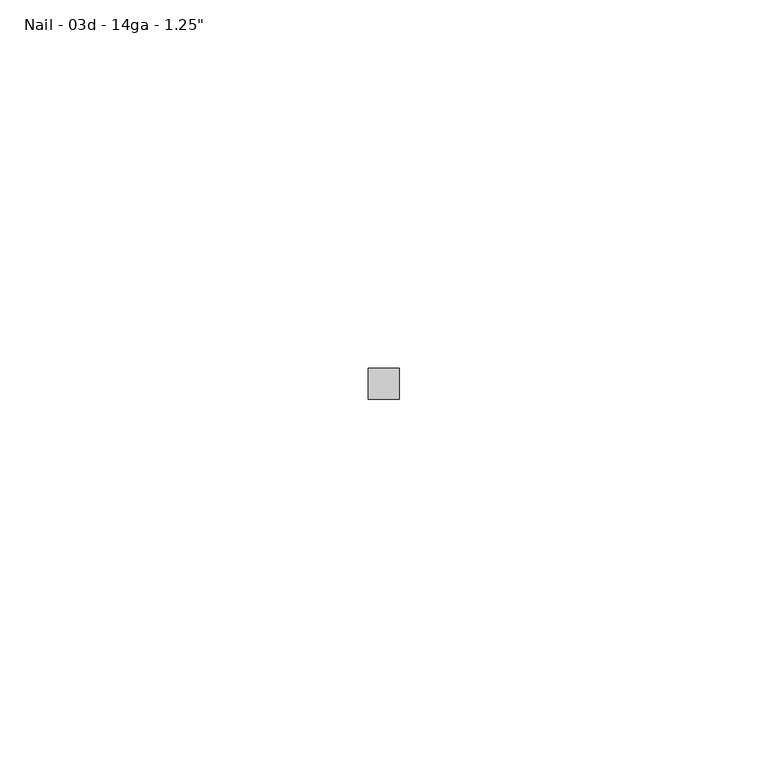
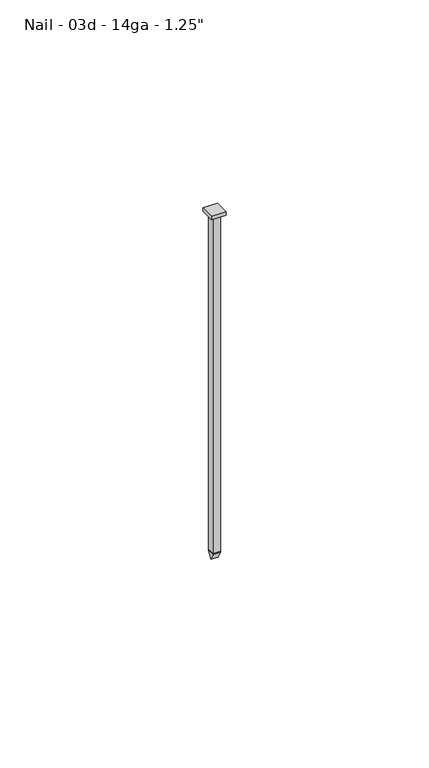
"""IFC4 building model written with IfcOpenShell, lengths in millimetres: fastener geometry."""

import ifcopenshell
import ifcopenshell.guid

model = None  # the IFC model being written
_history = None  # IfcOwnerHistory: only IFC2X3 demands one
_inside = {}  # id of a spatial element -> (the spatial element, [elements in it])
_under = {}  # id of a project, library or spatial element -> (it, [spatial elements below it])
_declared = {}  # id of a project -> (the project, [libraries it declares])
_typed = {}  # id of a type object -> (the type object, [elements of that type])
_made_of = {}  # id of a material, layer set ... -> (it, [elements and type objects made of it])


def new_model(schema):
    """Start an empty IFC model of exactly this schema.

    Asked for "IFC4X3", IfcOpenShell would pick the latest addendum, in which some entities
    have other attributes; the version numbers below select the first issue.
    IFC2X3 requires an IfcOwnerHistory on every rooted entity: one is made here for all.
    """
    global model, _history
    if schema == "IFC4X3":
        model = ifcopenshell.file(schema_version=(4, 3, 0, 0))
    else:
        model = ifcopenshell.file(schema=schema)
    _inside.clear()
    _under.clear()
    _declared.clear()
    _typed.clear()
    _made_of.clear()
    _history = None
    if model.schema == "IFC2X3":
        org = make("IfcOrganization", Name="unknown")
        user = make(
            "IfcPersonAndOrganization",
            ThePerson=make("IfcPerson", FamilyName="unknown"),
            TheOrganization=org,
        )
        app = make(
            "IfcApplication",
            ApplicationDeveloper=org,
            Version="unknown",
            ApplicationFullName="unknown",
            ApplicationIdentifier="unknown",
        )
        _history = make(
            "IfcOwnerHistory",
            OwningUser=user,
            OwningApplication=app,
            ChangeAction="ADDED",
            CreationDate=0,
        )
    return model


def make(cls, **values):
    """One entity of the class cls with the attributes given. An attribute that is None is left unset."""
    return model.create_entity(
        cls, **{name: value for name, value in values.items() if value is not None}
    )


def rooted(cls, **values):
    """An entity with a GlobalId (a new one), such as an element, a storey or a relation."""
    return make(cls, GlobalId=ifcopenshell.guid.new(), OwnerHistory=_history, **values)


def si_unit(unit_type, name, prefix=None):
    """IfcSIUnit, for example si_unit("LENGTHUNIT", "METRE", prefix="MILLI")."""
    return make("IfcSIUnit", UnitType=unit_type, Prefix=prefix, Name=name)


def assignment(units):
    """IfcUnitAssignment: the units of a project."""
    return None if units is None else make("IfcUnitAssignment", Units=units)


def point(xyz):
    """IfcCartesianPoint."""
    return None if xyz is None else make("IfcCartesianPoint", Coordinates=xyz)


def direction(xyz):
    """IfcDirection."""
    return None if xyz is None else make("IfcDirection", DirectionRatios=xyz)


def frame(location, z_axis=None, x_axis=None):
    """IfcAxis2Placement3D, a coordinate frame: its origin and axes. An axis left out is left unset."""
    return make(
        "IfcAxis2Placement3D",
        Location=point(location),
        Axis=direction(z_axis),
        RefDirection=direction(x_axis),
    )


def origin():
    """The frame at (0, 0, 0) with its axes left unset."""
    return frame((0.0, 0.0, 0.0))


def origin_with_axes():
    """The frame at (0, 0, 0) with the z axis (0, 0, 1) and the x axis (1, 0, 0) written out."""
    return frame((0.0, 0.0, 0.0), z_axis=(0.0, 0.0, 1.0), x_axis=(1.0, 0.0, 0.0))


def place(relative_to, where):
    """IfcLocalPlacement: puts the frame where relative to a parent placement (None: the world)."""
    return make(
        "IfcLocalPlacement", PlacementRelTo=relative_to, RelativePlacement=where
    )


def context(
    kind, dimensions, precision=None, world=None, true_north=None, identifier=None
):
    """IfcGeometricRepresentationContext, for example the 3D "Model" context."""
    return make(
        "IfcGeometricRepresentationContext",
        ContextIdentifier=identifier,
        ContextType=kind,
        CoordinateSpaceDimension=dimensions,
        Precision=precision,
        WorldCoordinateSystem=world,
        TrueNorth=true_north,
    )


def project(units=None, contexts=None):
    """IfcProject with its units and contexts."""
    return rooted(
        "IfcProject",
        Name="project",
        RepresentationContexts=contexts,
        UnitsInContext=assignment(units),
    )


def spatial(cls, under=None, at=None, **own):
    """A site, building, storey or space (cls), placed at a placement, below another one or the project."""
    s = rooted(cls, ObjectPlacement=at, **own)
    if under is not None:
        _under.setdefault(under.id(), (under, []))[1].append(s)
    return s


def polyline(points):
    """IfcPolyline through the points."""
    return make("IfcPolyline", Points=[point(p) for p in points])


def outline(outer, holes=None, kind="AREA"):
    """IfcArbitraryClosedProfileDef: a profile drawn as a closed curve; with holes, ...WithVoids."""
    if holes is None:
        return make("IfcArbitraryClosedProfileDef", ProfileType=kind, OuterCurve=outer)
    return make(
        "IfcArbitraryProfileDefWithVoids",
        ProfileType=kind,
        OuterCurve=outer,
        InnerCurves=holes,
    )


def extrude(swept, where, along, depth):
    """IfcExtrudedAreaSolid: the profile swept, set in the frame where, extruded along a direction by depth."""
    return make(
        "IfcExtrudedAreaSolid",
        SweptArea=swept,
        Position=where,
        ExtrudedDirection=direction(along),
        Depth=depth,
    )


def shape(context_of_items, identifier, shape_type, items):
    """IfcShapeRepresentation: the items that make up one representation, for example the "Body"."""
    return make(
        "IfcShapeRepresentation",
        ContextOfItems=context_of_items,
        RepresentationIdentifier=identifier,
        RepresentationType=shape_type,
        Items=items,
    )


def source(mapping_origin, context_of_items, identifier, shape_type, items):
    """IfcRepresentationMap: a shape defined once, which mapped items show again and again."""
    return make(
        "IfcRepresentationMap",
        MappingOrigin=mapping_origin,
        MappedRepresentation=shape(context_of_items, identifier, shape_type, items),
    )


def transform(
    local_origin,
    x_axis=None,
    y_axis=None,
    z_axis=None,
    scale=None,
    scale2=None,
    scale3=None,
    uniform=True,
):
    """IfcCartesianTransformationOperator3D, or its non-uniform kind. x_axis, y_axis, z_axis: its Axis1, 2, 3."""
    if uniform:
        return make(
            "IfcCartesianTransformationOperator3D",
            Axis1=direction(x_axis),
            Axis2=direction(y_axis),
            LocalOrigin=point(local_origin),
            Scale=scale,
            Axis3=direction(z_axis),
        )
    return make(
        "IfcCartesianTransformationOperator3DnonUniform",
        Axis1=direction(x_axis),
        Axis2=direction(y_axis),
        LocalOrigin=point(local_origin),
        Scale=scale,
        Axis3=direction(z_axis),
        Scale2=scale2,
        Scale3=scale3,
    )


def mapped(mapping_source, mapping_target):
    """IfcMappedItem: shows the shape of a source again, moved by a transform."""
    return make(
        "IfcMappedItem", MappingSource=mapping_source, MappingTarget=mapping_target
    )


def made_of(thing, what):
    """Note that an element or type object is made of a material, layer set ...; save() writes the relation."""
    if what is not None:
        _made_of.setdefault(what.id(), (what, []))[1].append(thing)
    return thing


def element(
    cls,
    number,
    at=None,
    inside=None,
    cuts=None,
    type_object=None,
    material=None,
    context=None,
    identifier="Body",
    shape_type=None,
    held_by="IfcProductDefinitionShape",
    body=None,
    shapes=None,
    **own,
):
    """One element of the class cls, such as IfcWall. Its Tag is "e" and its number.

    at: its placement. inside: the storey or other place that contains it. cuts: it is an
    opening in that element (IfcRelVoidsElement). A single representation is given by context,
    identifier, shape_type and body (its items); several are given by shapes. held_by: the class
    of the entity that holds the representations. save() writes the other relations.
    """
    e = rooted(cls, Tag="e%d" % number, ObjectPlacement=at, **own)
    if body is not None:
        shapes = [shape(context, identifier, shape_type, body)]
    if shapes is not None:
        e.Representation = make(held_by, Representations=shapes)
    if inside is not None:
        _inside.setdefault(inside.id(), (inside, []))[1].append(e)
    if cuts is not None:
        rooted(
            "IfcRelVoidsElement", RelatingBuildingElement=cuts, RelatedOpeningElement=e
        )
    if type_object is not None:
        _typed.setdefault(type_object.id(), (type_object, []))[1].append(e)
    return made_of(e, material)


def aggregate(whole, parts):
    """IfcRelAggregates: a whole, such as a stair, and the parts it consists of."""
    return rooted("IfcRelAggregates", RelatingObject=whole, RelatedObjects=parts)


def save(model, path):
    """Write the relations noted so far, then the file.

    IfcRelAggregates (storeys below a building ...), IfcRelContainedInSpatialStructure (elements
    in a storey), IfcRelDefinesByType, IfcRelAssociatesMaterial and IfcRelDeclares: one each for
    every whole, place, type object, material and project.
    """
    for whole, parts in _under.values():
        aggregate(whole, parts)
    for where, things in _inside.values():
        rooted(
            "IfcRelContainedInSpatialStructure",
            RelatedElements=things,
            RelatingStructure=where,
        )
    for kind, things in _typed.values():
        rooted("IfcRelDefinesByType", RelatedObjects=things, RelatingType=kind)
    for what, things in _made_of.values():
        rooted("IfcRelAssociatesMaterial", RelatedObjects=things, RelatingMaterial=what)
    for by, libraries in _declared.values():
        rooted("IfcRelDeclares", RelatingContext=by, RelatedDefinitions=libraries)
    model.write(path)


def fastener_3689d9c7(model_context):
    return source(origin(), model_context, "Body", "SweptSolid", [
        extrude(outline(polyline([(0.0, -103.7082), (-1.0541, -101.6), (1.0541, -101.6), (0.0, -103.7082)])), frame((-1.0541, 0.0, 0.0), z_axis=(1.0, 0.0, 0.0), x_axis=(0.0, 1.0, 0.0)), (0.0, 0.0, 1.0), 2.1082),
        extrude(outline(polyline([(-2.1082, -2.1082), (-2.1082, 2.1082), (2.1082, 2.1082), (2.1082, -2.1082), (-2.1082, -2.1082)])), origin_with_axes(), (0.0, 0.0, 1.0), 1.0541),
        extrude(outline(polyline([(-1.0541, 1.0541), (1.0541, 1.0541), (1.0541, -1.0541), (-1.0541, -1.0541), (-1.0541, 1.0541)])), frame((0.0, 0.0, -101.6), z_axis=(0.0, 0.0, 1.0), x_axis=(1.0, 0.0, 0.0)), (0.0, 0.0, 1.0), 101.6),
    ])


if __name__ == "__main__":
    model = new_model("IFC4")
    model_context = context("Model", 3, world=origin())
    ifc_project = project(units=[si_unit("LENGTHUNIT", "METRE", prefix="MILLI")], contexts=[model_context])
    site = spatial("IfcSite", under=ifc_project)
    building = spatial("IfcBuilding", under=site)
    placement = place(None, origin())
    fastener_shape = fastener_3689d9c7(model_context)
    element("IfcFastener", 1, ObjectType="060523 - W_P_C - Fastenings - Generic - SQUARE : Nail - 03d - 14ga - 1.25\"", at=placement, inside=building, context=model_context, shape_type="MappedRepresentation", body=[
        mapped(fastener_shape, transform((0.0, 0.0, 0.0), x_axis=(1.0, 0.0, 0.0), y_axis=(0.0, 1.0, 0.0), z_axis=(0.0, 0.0, 1.0))),
    ])
    save(model, "model.ifc")

# Revit data of these elements
# Type "060523 - W_P_C - Fastenings - Generic - SQUARE : Nail - 03d - 14ga - 1.25\""
#   Washer_Thickness = 0' - 0.00333"
#   Washer Radius = 0' - 0.0515"
#   Washer Offset - Head = 0' - 0"
#   Washer Offset = 0' - 0"
#   Thickness_of_Substrate [instance default] = 0' - 1"
#   Side = 0' - 0 37/64"
#   Radius = 0' - 0.0415"
#   Length [instance default] = 0' - 1 1/4"
#   Head Size = 0' - 1"
#   Head Radius = 0' - 0 1/2"
#   Head Height = 0' - 0.01"
#   Double Diameter = 0' - 0.166"
#   Diameter = 0' - 0.083"
#   Default Elevation = 4' - 0"
#   Washer_Nut_Visibility = no
#   Washer_Head_Visibility = no
#   Round_Head_Visibility = yes
#   Point Visibility = yes
#   Nut_Visibility = no
#   Hex_Head_Visiblilty = no
#   Washer Material = none
#   Bolt Material (Size) = AT SILL - FASTENER AT 24" O.C.
# Element 1 (IfcFastener, "060523 - W_P_C - Fastenings - Generic - SQUARE : Nail - 03d - 14ga - 1.25\"")
#   Length = 0' - 4"
# Materials
#   "AT SILL - FASTENER AT 24\" O.C.": class "Generic", colour RGB 120 120 120, transparency 0, Cost = 0
